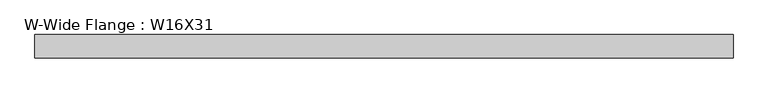
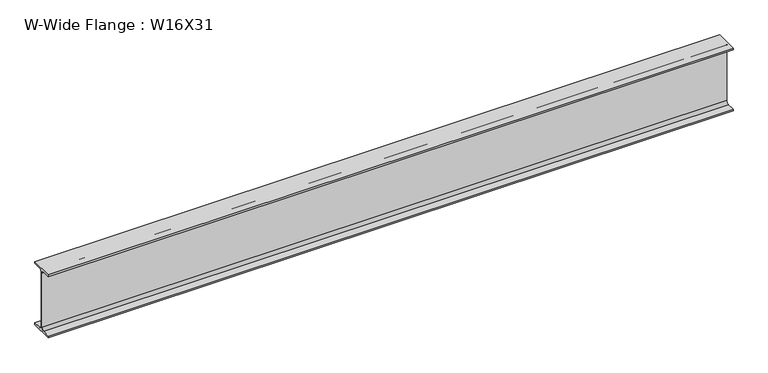
"""IFC4 building model written with IfcOpenShell, lengths in millimetres: beam geometry, W-Wide Flange : W16X31."""

from ifc_helpers import new_model, si_unit, point, frame, frame_2d, origin, place, context, project, spatial, polyline, circle_curve, trimmed, segment, composite_curve, outline, extrude, source, transform, mapped, element, save


def w_wide_flange_w16x31_b13c45c6(model_context):
    return source(origin(), model_context, "Body", "SweptSolid", [
        extrude(outline(composite_curve([segment(polyline([(70.231, -190.754), (70.231, -201.93), (-70.231, -201.93), (-70.231, -190.754), (-20.8915, -190.754)]), True, "CONTINUOUS"), segment(trimmed(circle_curve(frame_2d((-20.8915, -173.355)), 17.399), [point((-20.8915, -190.754))], [point((-3.4925, -173.355))], True, "CARTESIAN"), True, "CONTINUOUS"), segment(polyline([(-3.4925, -173.355), (-3.4925, 173.355)]), True, "CONTINUOUS"), segment(trimmed(circle_curve(frame_2d((-20.8915, 173.355)), 17.399), [point((-3.4925, 173.355))], [point((-20.8915, 190.754))], True, "CARTESIAN"), True, "CONTINUOUS"), segment(polyline([(-20.8915, 190.754), (-70.231, 190.754), (-70.231, 201.93), (70.231, 201.93), (70.231, 190.754), (20.8915, 190.754)]), True, "CONTINUOUS"), segment(trimmed(circle_curve(frame_2d((20.8915, 173.355)), 17.399), [point((20.8915, 190.754))], [point((3.4925, 173.355))], True, "CARTESIAN"), True, "CONTINUOUS"), segment(polyline([(3.4925, 173.355), (3.4925, -173.355)]), True, "CONTINUOUS"), segment(trimmed(circle_curve(frame_2d((20.8915, -173.355)), 17.399), [point((3.4925, -173.355))], [point((20.8915, -190.754))], True, "CARTESIAN"), True, "CONTINUOUS"), segment(polyline([(20.8915, -190.754), (70.231, -190.754)]), True, "CONTINUOUS")], self_intersect=False)), frame((-2082.8, 0.0, 0.0), z_axis=(1.0, 0.0, 0.0), x_axis=(0.0, 1.0, 0.0)), (0.0, 0.0, 1.0), 4165.6),
    ])


if __name__ == "__main__":
    model = new_model("IFC4")
    model_context = context("Model", 3, world=origin())
    ifc_project = project(units=[si_unit("LENGTHUNIT", "METRE", prefix="MILLI")], contexts=[model_context])
    site = spatial("IfcSite", under=ifc_project)
    building = spatial("IfcBuilding", under=site)
    placement = place(None, origin())
    w_wide_flange_w16x31_shape = w_wide_flange_w16x31_b13c45c6(model_context)
    element("IfcBeam", 1, ObjectType="W-Wide Flange : W16X31", at=placement, inside=building, context=model_context, shape_type="MappedRepresentation", body=[
        mapped(w_wide_flange_w16x31_shape, transform((0.0, 0.0, 0.0), x_axis=(1.0, 0.0, 0.0), y_axis=(0.0, 1.0, 0.0), z_axis=(0.0, 0.0, 1.0))),
    ])
    save(model, "model.ifc")

# Revit data of these elements
# Type "W-Wide Flange : W16X31"
#   Assembly Code = "B10"
#   W = 31
#   Length [instance default] = 5' - 0"
#   bf = 0' - 5.53"
#   d = 1' - 3.9"
#   k = 0' - 1 1/8"
#   k2 = 0' - 0.685"
#   tf = 0' - 0.44"
#   tw = 0' - 0.275"
#   A = 0.0634028 SF
#   Structural Material [instance default] = Steel ASTM A992
# Element 1 (IfcBeam, "W-Wide Flange : W16X31")
#   Materials on its faces: "Steel ASTM A992"
# Materials
#   "Steel ASTM A992": class "Metal", colour RGB 199 199 199, transparency 0, Description = "Structural steel 50ksi", Cost = 0
